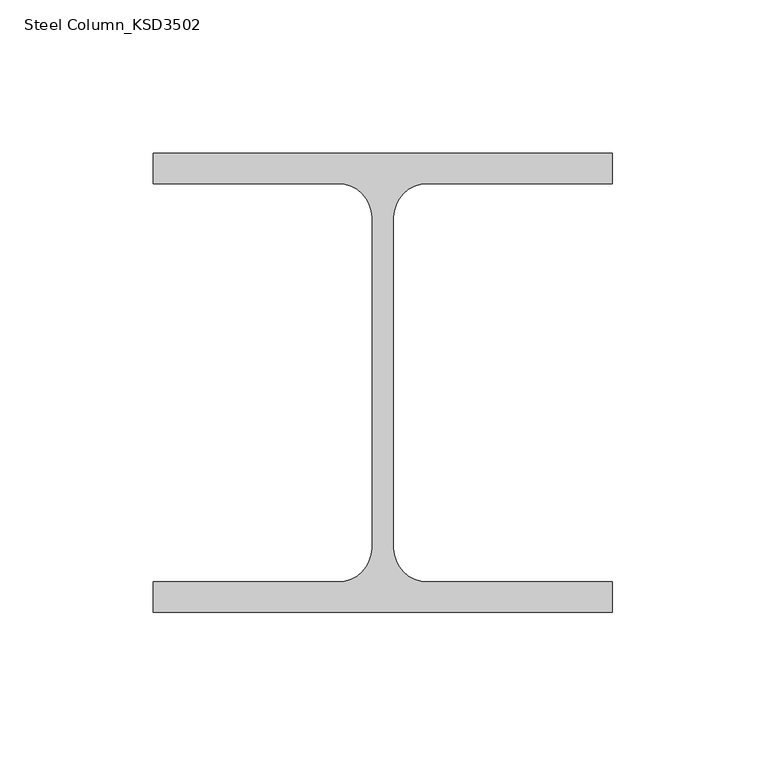
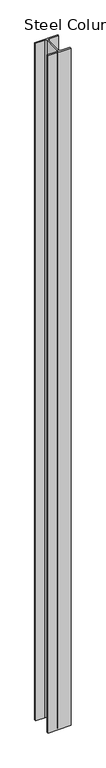
"""IFC4 building model written with IfcOpenShell, lengths in millimetres: column geometry, Steel Column_KSD3502 : H_SC_ASC_H-150×150x7x10."""

from ifc_helpers import new_model, si_unit, point, frame, frame_2d, origin, place, context, project, spatial, polyline, circle_curve, trimmed, segment, composite_curve, outline, extrude, source, transform, mapped, element, save


def steel_column_ksd3502_23aad0d9(model_context):
    return source(origin(), model_context, "Body", "SweptSolid", [
        extrude(outline(composite_curve([segment(polyline([(75.0, 75.0), (75.0, 65.0), (14.5, 65.0)]), True, "CONTINUOUS"), segment(trimmed(circle_curve(frame_2d((14.5, 54.0)), 11.0), [point((14.5, 65.0))], [point((3.5, 54.0))], True, "CARTESIAN"), True, "CONTINUOUS"), segment(polyline([(3.5, 54.0), (3.5, -54.0)]), True, "CONTINUOUS"), segment(trimmed(circle_curve(frame_2d((14.5, -54.0)), 11.0), [point((3.5, -54.0))], [point((14.5, -65.0))], True, "CARTESIAN"), True, "CONTINUOUS"), segment(polyline([(14.5, -65.0), (75.0, -65.0), (75.0, -75.0), (-75.0, -75.0), (-75.0, -65.0), (-14.5, -65.0)]), True, "CONTINUOUS"), segment(trimmed(circle_curve(frame_2d((-14.5, -54.0)), 11.0), [point((-14.5, -65.0))], [point((-3.5, -54.0))], True, "CARTESIAN"), True, "CONTINUOUS"), segment(polyline([(-3.5, -54.0), (-3.5, 54.0)]), True, "CONTINUOUS"), segment(trimmed(circle_curve(frame_2d((-14.5, 54.0)), 11.0), [point((-3.5, 54.0))], [point((-14.5, 65.0))], True, "CARTESIAN"), True, "CONTINUOUS"), segment(polyline([(-14.5, 65.0), (-75.0, 65.0), (-75.0, 75.0), (75.0, 75.0)]), True, "CONTINUOUS")], self_intersect=False)), frame((0.0, 0.0, 12299.9720055), z_axis=(0.0, 0.0, 1.0), x_axis=(1.0, 0.0, 0.0)), (0.0, 0.0, 1.0), 4650.0),
    ])


if __name__ == "__main__":
    model = new_model("IFC4")
    model_context = context("Model", 3, world=origin())
    ifc_project = project(units=[si_unit("LENGTHUNIT", "METRE", prefix="MILLI")], contexts=[model_context])
    site = spatial("IfcSite", under=ifc_project)
    building = spatial("IfcBuilding", under=site)
    placement = place(None, origin())
    steel_column_ksd3502_shape = steel_column_ksd3502_23aad0d9(model_context)
    element("IfcColumn", 1, ObjectType="Steel Column_KSD3502 : H_SC_ASC_H-150×150x7x10", at=placement, inside=building, context=model_context, shape_type="MappedRepresentation", body=[
        mapped(steel_column_ksd3502_shape, transform((0.0, 0.0, 0.0), x_axis=(1.0, 0.0, 0.0), y_axis=(0.0, 1.0, 0.0), z_axis=(0.0, 0.0, 1.0))),
    ])
    save(model, "model.ifc")

# Revit data of these elements
# Type "Steel Column_KSD3502 : H_SC_ASC_H-150×150x7x10"
#   Width = 15.0 cm
#   Web Thickness = 0.7 cm
#   Web Fillet = 1.1 cm
#   Warping Constant = 27562.5 cm⁶
#   Torsional Moment of Inertia = 11.6007 cm⁴
#   Section Area = 40.14 cm²
#   Plastic Modulus weak axis = 115.0 cm³
#   Plastic Modulus strong axis = 246.0 cm³
#   Perimeter = 1.27 m²/m
#   Nominal Weight = 31.50 kgf/m
#   Moment of Inertia weak axis = 563.00 cm⁴
#   Moment of Inertia strong axis = 1640.00 cm⁴
#   Height = 15.0 cm
#   Flange Thickness = 1.0 cm
#   Elastic Modulus weak axis = 75.1 cm³
#   Elastic Modulus strong axis = 219.0 cm³
#   Centroid Vertical = 7.5 cm
#   Centroid Horizontal = 7.5 cm
#   Bolt Spacing = 13.97 cm
#   Structural Material [instance default] = Steel, 45-345
#   Section Name Key = ""
#   Assembly Code = ""
# Element 1 (IfcColumn, "Steel Column_KSD3502 : H_SC_ASC_H-150×150x7x10")
#   Structural Material = none
# Materials
#   "Steel, 45-345": class "Metal", colour RGB 189 187 185, transparency 0, Description = "Steel 345 MPa", Cost = 0
